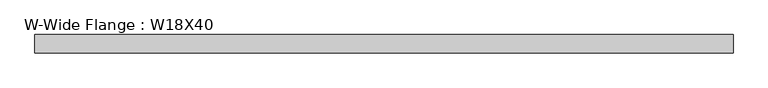
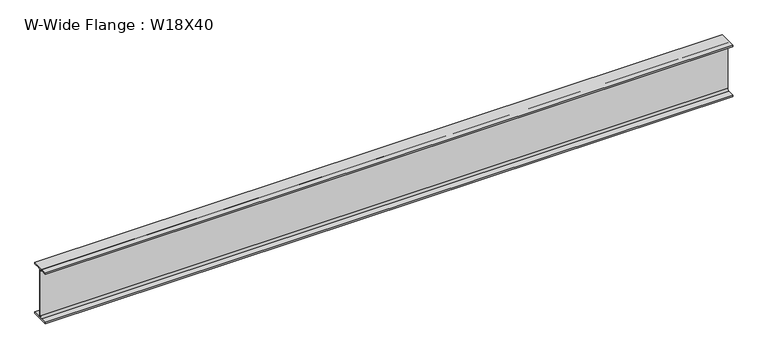
"""IFC4 building model written with IfcOpenShell, lengths in millimetres: beam geometry, W-Wide Flange : W18X40."""

from ifc_helpers import new_model, si_unit, point, frame, frame_2d, origin, place, context, project, spatial, polyline, circle_curve, trimmed, segment, composite_curve, outline, extrude, source, transform, mapped, element, save


def w_wide_flange_w18x40_3d1222e0(model_context):
    return source(origin(), model_context, "Body", "SweptSolid", [
        extrude(outline(composite_curve([segment(polyline([(76.454, -213.995), (76.454, -227.33), (-76.454, -227.33), (-76.454, -213.995), (-20.828, -213.995)]), True, "CONTINUOUS"), segment(trimmed(circle_curve(frame_2d((-20.828, -197.1675)), 16.8275), [point((-20.828, -213.995))], [point((-4.0005, -197.1675))], True, "CARTESIAN"), True, "CONTINUOUS"), segment(polyline([(-4.0005, -197.1675), (-4.0005, 197.1675)]), True, "CONTINUOUS"), segment(trimmed(circle_curve(frame_2d((-20.828, 197.1675)), 16.8275), [point((-4.0005, 197.1675))], [point((-20.828, 213.995))], True, "CARTESIAN"), True, "CONTINUOUS"), segment(polyline([(-20.828, 213.995), (-76.454, 213.995), (-76.454, 227.33), (76.454, 227.33), (76.454, 213.995), (20.828, 213.995)]), True, "CONTINUOUS"), segment(trimmed(circle_curve(frame_2d((20.828, 197.1675)), 16.8275), [point((20.828, 213.995))], [point((4.0005, 197.1675))], True, "CARTESIAN"), True, "CONTINUOUS"), segment(polyline([(4.0005, 197.1675), (4.0005, -197.1675)]), True, "CONTINUOUS"), segment(trimmed(circle_curve(frame_2d((20.828, -197.1675)), 16.8275), [point((4.0005, -197.1675))], [point((20.828, -213.995))], True, "CARTESIAN"), True, "CONTINUOUS"), segment(polyline([(20.828, -213.995), (76.454, -213.995)]), True, "CONTINUOUS")], self_intersect=False)), frame((-2881.63, 0.0, 0.0), z_axis=(1.0, 0.0, 0.0), x_axis=(0.0, 1.0, 0.0)), (0.0, 0.0, 1.0), 5758.18),
    ])


if __name__ == "__main__":
    model = new_model("IFC4")
    model_context = context("Model", 3, world=origin())
    ifc_project = project(units=[si_unit("LENGTHUNIT", "METRE", prefix="MILLI")], contexts=[model_context])
    site = spatial("IfcSite", under=ifc_project)
    building = spatial("IfcBuilding", under=site)
    placement = place(None, origin())
    w_wide_flange_w18x40_shape = w_wide_flange_w18x40_3d1222e0(model_context)
    element("IfcBeam", 1, ObjectType="W-Wide Flange : W18X40", at=placement, inside=building, context=model_context, shape_type="MappedRepresentation", body=[
        mapped(w_wide_flange_w18x40_shape, transform((0.0, 0.0, 0.0), x_axis=(1.0, 0.0, 0.0), y_axis=(0.0, 1.0, 0.0), z_axis=(0.0, 0.0, 1.0))),
    ])
    save(model, "model.ifc")

# Revit data of these elements
# Type "W-Wide Flange : W18X40"
#   Assembly Code = "B10"
#   W = 40
#   Length [instance default] = 5' - 0"
#   bf = 0' - 6.02"
#   d = 1' - 5.9"
#   k = 0' - 1 3/16"
#   k2 = 0' - 0.6625"
#   tf = 0' - 0.525"
#   tw = 0' - 0.315"
#   A = 0.0819444 SF
#   Structural Material [instance default] = Steel ASTM A992
# Element 1 (IfcBeam, "W-Wide Flange : W18X40")
#   Materials on its faces: "Steel ASTM A992"
# Materials
#   "Steel ASTM A992": class "Metal", colour RGB 199 199 199, transparency 0, Description = "Structural steel 50ksi", Cost = 0
